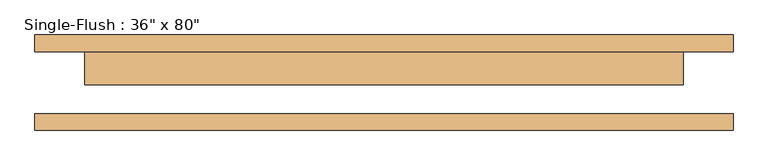
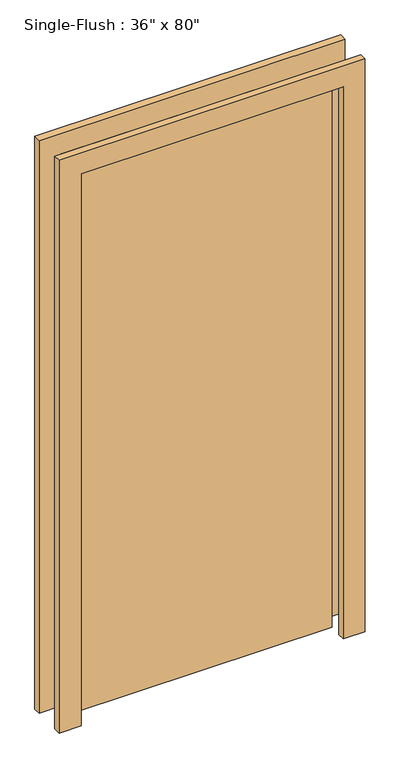
"""IFC4 building model written with IfcOpenShell, lengths in millimetres: door geometry."""

import ifcopenshell
import ifcopenshell.guid

model = None  # the IFC model being written
_history = None  # IfcOwnerHistory: only IFC2X3 demands one
_inside = {}  # id of a spatial element -> (the spatial element, [elements in it])
_under = {}  # id of a project, library or spatial element -> (it, [spatial elements below it])
_declared = {}  # id of a project -> (the project, [libraries it declares])
_typed = {}  # id of a type object -> (the type object, [elements of that type])
_made_of = {}  # id of a material, layer set ... -> (it, [elements and type objects made of it])


def new_model(schema):
    """Start an empty IFC model of exactly this schema.

    Asked for "IFC4X3", IfcOpenShell would pick the latest addendum, in which some entities
    have other attributes; the version numbers below select the first issue.
    IFC2X3 requires an IfcOwnerHistory on every rooted entity: one is made here for all.
    """
    global model, _history
    if schema == "IFC4X3":
        model = ifcopenshell.file(schema_version=(4, 3, 0, 0))
    else:
        model = ifcopenshell.file(schema=schema)
    _inside.clear()
    _under.clear()
    _declared.clear()
    _typed.clear()
    _made_of.clear()
    _history = None
    if model.schema == "IFC2X3":
        org = make("IfcOrganization", Name="unknown")
        user = make(
            "IfcPersonAndOrganization",
            ThePerson=make("IfcPerson", FamilyName="unknown"),
            TheOrganization=org,
        )
        app = make(
            "IfcApplication",
            ApplicationDeveloper=org,
            Version="unknown",
            ApplicationFullName="unknown",
            ApplicationIdentifier="unknown",
        )
        _history = make(
            "IfcOwnerHistory",
            OwningUser=user,
            OwningApplication=app,
            ChangeAction="ADDED",
            CreationDate=0,
        )
    return model


def make(cls, **values):
    """One entity of the class cls with the attributes given. An attribute that is None is left unset."""
    return model.create_entity(
        cls, **{name: value for name, value in values.items() if value is not None}
    )


def rooted(cls, **values):
    """An entity with a GlobalId (a new one), such as an element, a storey or a relation."""
    return make(cls, GlobalId=ifcopenshell.guid.new(), OwnerHistory=_history, **values)


def si_unit(unit_type, name, prefix=None):
    """IfcSIUnit, for example si_unit("LENGTHUNIT", "METRE", prefix="MILLI")."""
    return make("IfcSIUnit", UnitType=unit_type, Prefix=prefix, Name=name)


def assignment(units):
    """IfcUnitAssignment: the units of a project."""
    return None if units is None else make("IfcUnitAssignment", Units=units)


def point(xyz):
    """IfcCartesianPoint."""
    return None if xyz is None else make("IfcCartesianPoint", Coordinates=xyz)


def direction(xyz):
    """IfcDirection."""
    return None if xyz is None else make("IfcDirection", DirectionRatios=xyz)


def frame(location, z_axis=None, x_axis=None):
    """IfcAxis2Placement3D, a coordinate frame: its origin and axes. An axis left out is left unset."""
    return make(
        "IfcAxis2Placement3D",
        Location=point(location),
        Axis=direction(z_axis),
        RefDirection=direction(x_axis),
    )


def origin():
    """The frame at (0, 0, 0) with its axes left unset."""
    return frame((0.0, 0.0, 0.0))


def origin_with_axes():
    """The frame at (0, 0, 0) with the z axis (0, 0, 1) and the x axis (1, 0, 0) written out."""
    return frame((0.0, 0.0, 0.0), z_axis=(0.0, 0.0, 1.0), x_axis=(1.0, 0.0, 0.0))


def place(relative_to, where):
    """IfcLocalPlacement: puts the frame where relative to a parent placement (None: the world)."""
    return make(
        "IfcLocalPlacement", PlacementRelTo=relative_to, RelativePlacement=where
    )


def context(
    kind, dimensions, precision=None, world=None, true_north=None, identifier=None
):
    """IfcGeometricRepresentationContext, for example the 3D "Model" context."""
    return make(
        "IfcGeometricRepresentationContext",
        ContextIdentifier=identifier,
        ContextType=kind,
        CoordinateSpaceDimension=dimensions,
        Precision=precision,
        WorldCoordinateSystem=world,
        TrueNorth=true_north,
    )


def project(units=None, contexts=None):
    """IfcProject with its units and contexts."""
    return rooted(
        "IfcProject",
        Name="project",
        RepresentationContexts=contexts,
        UnitsInContext=assignment(units),
    )


def spatial(cls, under=None, at=None, **own):
    """A site, building, storey or space (cls), placed at a placement, below another one or the project."""
    s = rooted(cls, ObjectPlacement=at, **own)
    if under is not None:
        _under.setdefault(under.id(), (under, []))[1].append(s)
    return s


def polyline(points):
    """IfcPolyline through the points."""
    return make("IfcPolyline", Points=[point(p) for p in points])


def outline(outer, holes=None, kind="AREA"):
    """IfcArbitraryClosedProfileDef: a profile drawn as a closed curve; with holes, ...WithVoids."""
    if holes is None:
        return make("IfcArbitraryClosedProfileDef", ProfileType=kind, OuterCurve=outer)
    return make(
        "IfcArbitraryProfileDefWithVoids",
        ProfileType=kind,
        OuterCurve=outer,
        InnerCurves=holes,
    )


def extrude(swept, where, along, depth):
    """IfcExtrudedAreaSolid: the profile swept, set in the frame where, extruded along a direction by depth."""
    return make(
        "IfcExtrudedAreaSolid",
        SweptArea=swept,
        Position=where,
        ExtrudedDirection=direction(along),
        Depth=depth,
    )


def shape(context_of_items, identifier, shape_type, items):
    """IfcShapeRepresentation: the items that make up one representation, for example the "Body"."""
    return make(
        "IfcShapeRepresentation",
        ContextOfItems=context_of_items,
        RepresentationIdentifier=identifier,
        RepresentationType=shape_type,
        Items=items,
    )


def source(mapping_origin, context_of_items, identifier, shape_type, items):
    """IfcRepresentationMap: a shape defined once, which mapped items show again and again."""
    return make(
        "IfcRepresentationMap",
        MappingOrigin=mapping_origin,
        MappedRepresentation=shape(context_of_items, identifier, shape_type, items),
    )


def transform(
    local_origin,
    x_axis=None,
    y_axis=None,
    z_axis=None,
    scale=None,
    scale2=None,
    scale3=None,
    uniform=True,
):
    """IfcCartesianTransformationOperator3D, or its non-uniform kind. x_axis, y_axis, z_axis: its Axis1, 2, 3."""
    if uniform:
        return make(
            "IfcCartesianTransformationOperator3D",
            Axis1=direction(x_axis),
            Axis2=direction(y_axis),
            LocalOrigin=point(local_origin),
            Scale=scale,
            Axis3=direction(z_axis),
        )
    return make(
        "IfcCartesianTransformationOperator3DnonUniform",
        Axis1=direction(x_axis),
        Axis2=direction(y_axis),
        LocalOrigin=point(local_origin),
        Scale=scale,
        Axis3=direction(z_axis),
        Scale2=scale2,
        Scale3=scale3,
    )


def mapped(mapping_source, mapping_target):
    """IfcMappedItem: shows the shape of a source again, moved by a transform."""
    return make(
        "IfcMappedItem", MappingSource=mapping_source, MappingTarget=mapping_target
    )


def made_of(thing, what):
    """Note that an element or type object is made of a material, layer set ...; save() writes the relation."""
    if what is not None:
        _made_of.setdefault(what.id(), (what, []))[1].append(thing)
    return thing


def element(
    cls,
    number,
    at=None,
    inside=None,
    cuts=None,
    type_object=None,
    material=None,
    context=None,
    identifier="Body",
    shape_type=None,
    held_by="IfcProductDefinitionShape",
    body=None,
    shapes=None,
    **own,
):
    """One element of the class cls, such as IfcWall. Its Tag is "e" and its number.

    at: its placement. inside: the storey or other place that contains it. cuts: it is an
    opening in that element (IfcRelVoidsElement). A single representation is given by context,
    identifier, shape_type and body (its items); several are given by shapes. held_by: the class
    of the entity that holds the representations. save() writes the other relations.
    """
    e = rooted(cls, Tag="e%d" % number, ObjectPlacement=at, **own)
    if body is not None:
        shapes = [shape(context, identifier, shape_type, body)]
    if shapes is not None:
        e.Representation = make(held_by, Representations=shapes)
    if inside is not None:
        _inside.setdefault(inside.id(), (inside, []))[1].append(e)
    if cuts is not None:
        rooted(
            "IfcRelVoidsElement", RelatingBuildingElement=cuts, RelatedOpeningElement=e
        )
    if type_object is not None:
        _typed.setdefault(type_object.id(), (type_object, []))[1].append(e)
    return made_of(e, material)


def aggregate(whole, parts):
    """IfcRelAggregates: a whole, such as a stair, and the parts it consists of."""
    return rooted("IfcRelAggregates", RelatingObject=whole, RelatedObjects=parts)


def save(model, path):
    """Write the relations noted so far, then the file.

    IfcRelAggregates (storeys below a building ...), IfcRelContainedInSpatialStructure (elements
    in a storey), IfcRelDefinesByType, IfcRelAssociatesMaterial and IfcRelDeclares: one each for
    every whole, place, type object, material and project.
    """
    for whole, parts in _under.values():
        aggregate(whole, parts)
    for where, things in _inside.values():
        rooted(
            "IfcRelContainedInSpatialStructure",
            RelatedElements=things,
            RelatingStructure=where,
        )
    for kind, things in _typed.values():
        rooted("IfcRelDefinesByType", RelatedObjects=things, RelatingType=kind)
    for what, things in _made_of.values():
        rooted("IfcRelAssociatesMaterial", RelatedObjects=things, RelatingMaterial=what)
    for by, libraries in _declared.values():
        rooted("IfcRelDeclares", RelatingContext=by, RelatedDefinitions=libraries)
    model.write(path)


def door_cf5a424f(model_context):
    return source(origin(), model_context, "Body", "SweptSolid", [
        extrude(outline(polyline([(2108.2, -533.4), (0.0, -533.4), (0.0, -457.2), (2032.0, -457.2), (2032.0, 457.2), (0.0, 457.2), (0.0, 533.4), (2108.2, 533.4), (2108.2, -533.4)])), frame((0.0, 47.625, 0.0), z_axis=(0.0, 1.0, 0.0), x_axis=(0.0, 0.0, 1.0)), (0.0, 0.0, 1.0), 25.4),
        extrude(outline(polyline([(2108.2, 533.4), (2108.2, -533.4), (0.0, -533.4), (0.0, -457.2), (2032.0, -457.2), (2032.0, 457.2), (0.0, 457.2), (0.0, 533.4), (2108.2, 533.4)])), frame((0.0, -73.025, 0.0), z_axis=(0.0, 1.0, 0.0), x_axis=(0.0, 0.0, 1.0)), (0.0, 0.0, 1.0), 25.4),
        extrude(outline(polyline([(457.2, -3.175), (-457.2, -3.175), (-457.2, 47.625), (457.2, 47.625), (457.2, -3.175)])), origin_with_axes(), (0.0, 0.0, 1.0), 2032.0),
    ])


if __name__ == "__main__":
    model = new_model("IFC4")
    model_context = context("Model", 3, world=origin())
    ifc_project = project(units=[si_unit("LENGTHUNIT", "METRE", prefix="MILLI")], contexts=[model_context])
    site = spatial("IfcSite", under=ifc_project)
    building = spatial("IfcBuilding", under=site)
    placement = place(None, origin())
    door_shape = door_cf5a424f(model_context)
    element("IfcDoor", 1, ObjectType="Single-Flush : 36\" x 80\"", at=placement, inside=building, context=model_context, shape_type="MappedRepresentation", body=[
        mapped(door_shape, transform((0.0, 0.0, 0.0), x_axis=(1.0, 0.0, 0.0), y_axis=(0.0, 1.0, 0.0), z_axis=(0.0, 0.0, 1.0))),
    ])
    save(model, "model.ifc")

# Revit data of these elements
# Type "Single-Flush : 36\" x 80\""
#   Type Mark = "6"
#   Assembly Code = "C1020"
#   Thickness = 50.8 mm
#   Height = 2032 mm
#   Trim Projection Ext = 25.4 mm
#   Trim Projection Int = 25.4 mm
#   Trim Width = 76.2 mm
#   Width = 914.4 mm
#   Door Material = Door - Panel
#   Frame Material = Door - Frame
#   Function = (empty or 0)
#   Wall Closure = (empty or 0)
# Element 1 (IfcDoor, "Single-Flush : 36\" x 80\"")
#   Materials on its faces: "Door - Frame", "Door - Panel"
# Materials
#   "Door - Panel": class "Wood", colour RGB 210 159 95, transparency 0
#   "Door - Frame": class "Miscellaneous", colour RGB 118 70 51, transparency 0
